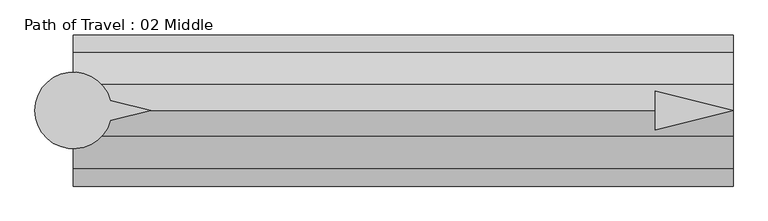
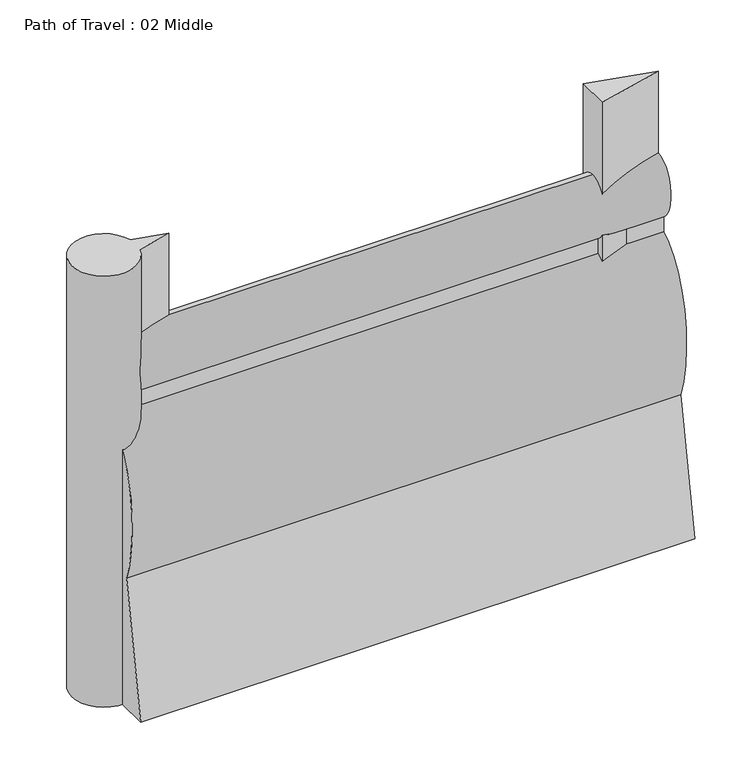
"""IFC4 building model written with IfcOpenShell, lengths in millimetres: proxy geometry, Path of Travel : 02 Middle."""

from ifc_helpers import new_model, si_unit, point, frame, frame_2d, origin, origin_with_axes, place, context, project, spatial, polyline, circle_curve, ellipse_curve, trimmed, segment, composite_curve, outline, extrude, source, transform, mapped, element, save
from ifc_brep_helpers import plane_surface, extruded_surface, advanced_brep


def path_of_travel_02_middle_c592e2b7(model_context):
    return source(origin(), model_context, "Body", "SolidModel", [
        advanced_brep(
        [(227.5554837, 0.0, 1727.2), (227.5554837, 42.9018657, 1436.6534209), (227.5554837, 42.9018657, 1363.4763406), (227.5554837, 184.1186263, 643.4144547), (227.5554837, 297.5699544, 0.0), (227.5554837, 145.6574193, 0.0), (227.5554837, 0.0, 584.2), (227.5554837, -145.6574193, 0.0), (227.5554837, -297.5699544, 0.0), (227.5554837, -184.1186263, 643.4144547), (227.5554837, -42.9018657, 1363.4763406), (227.5554837, -42.9018657, 1436.6534209), (2818.3554837, 0.0, 1727.2), (2818.3554837, -42.9018657, 1436.6534209), (2818.3554837, -42.9018657, 1363.4763406), (2818.3554837, -184.1186263, 643.4144547), (2818.3554837, -297.5699544, 0.0), (2818.3554837, -145.6574193, 0.0), (2818.3554837, 0.0, 584.2), (2818.3554837, 145.6574193, 0.0), (2818.3554837, 297.5699544, 0.0), (2818.3554837, 184.1186263, 643.4144547), (2818.3554837, 42.9018657, 1363.4763406), (2818.3554837, 42.9018657, 1436.6534209)],
        [
            (0, 1, ellipse_curve(frame((227.5554837, 0.0, 1574.8), z_axis=(-1.0, 0.0, 0.0), x_axis=(0.0, 0.0, 1.0)), 152.4, 101.6)),
            (1, 2),
            (2, 3, ellipse_curve(frame((227.5554837, 0.0, 914.4), z_axis=(-1.0, 0.0, 0.0), x_axis=(0.0, 0.0, -1.0)), 457.2, 228.6)),
            (3, 4),
            (4, 5),
            (5, 6),
            (6, 7),
            (7, 8),
            (8, 9),
            (9, 10, ellipse_curve(frame((227.5554837, 0.0, 914.4), z_axis=(-1.0, 0.0, 0.0), x_axis=(0.0, 0.0, -1.0)), 457.2, 228.6)),
            (10, 11),
            (11, 0, ellipse_curve(frame((227.5554837, 0.0, 1574.8), z_axis=(-1.0, 0.0, 0.0), x_axis=(0.0, 0.0, 1.0)), 152.4, 101.6)),
            (12, 13, ellipse_curve(frame((2818.3554837, 0.0, 1574.8), z_axis=(1.0, 0.0, 0.0), x_axis=(0.0, 0.0, 1.0)), 152.4, 101.6)),
            (13, 14),
            (14, 15, ellipse_curve(frame((2818.3554837, 0.0, 914.4), z_axis=(1.0, 0.0, 0.0), x_axis=(0.0, 0.0, -1.0)), 457.2, 228.6)),
            (15, 16),
            (16, 17),
            (17, 18),
            (18, 19),
            (19, 20),
            (20, 21),
            (21, 22, ellipse_curve(frame((2818.3554837, 0.0, 914.4), z_axis=(1.0, 0.0, 0.0), x_axis=(0.0, 0.0, -1.0)), 457.2, 228.6)),
            (22, 23),
            (23, 12, ellipse_curve(frame((2818.3554837, 0.0, 1574.8), z_axis=(1.0, 0.0, 0.0), x_axis=(0.0, 0.0, 1.0)), 152.4, 101.6)),
            (0, 12),
            (23, 1),
            (22, 2),
            (21, 3),
            (20, 4),
            (19, 5),
            (18, 6),
            (17, 7),
            (16, 8),
            (15, 9),
            (14, 10),
            (13, 11),
        ],
        [
            plane_surface(frame((227.5554837, 0.0, 0.0), z_axis=(-1.0, 0.0, 0.0), x_axis=(0.0, 0.0, 1.0))),
            plane_surface(frame((2818.3554837, 0.0, 0.0), z_axis=(1.0, 0.0, 0.0), x_axis=(0.0, 0.0, 1.0))),
            extruded_surface(trimmed(ellipse_curve(frame((2818.3554837, 0.0, 1574.8), z_axis=(-1.0, 0.0, 0.0), x_axis=(0.0, 0.0, 1.0)), 152.4, 101.6), [point((2818.3554837, 0.0, 1727.2))], [point((2818.3554837, 42.9018657, 1436.6534209))], True, "CARTESIAN"), (-2590.8, 0.0, 0.0), 2590.8),
            plane_surface(frame((227.5554837, 42.9018657, 1436.6534209), z_axis=(0.0, 1.0, 0.0), x_axis=(1.0, 0.0, 0.0))),
            extruded_surface(trimmed(ellipse_curve(frame((2818.3554837, 0.0, 914.4), z_axis=(-1.0, 0.0, 0.0), x_axis=(0.0, 0.0, -1.0)), 457.2, 228.6), [point((2818.3554837, 42.9018657, 1363.4763406))], [point((2818.3554837, 184.1186263, 643.4144547))], True, "CARTESIAN"), (-2590.8, 0.0, 0.0), 2590.8),
            plane_surface(frame((227.5554837, 184.1186263, 643.4144547), z_axis=(0.0, 0.9848077530122078, 0.1736481776669322), x_axis=(1.0, 0.0, 0.0))),
            plane_surface(frame((227.5554837, 297.5699544, 0.0), z_axis=(0.0, 0.0, -1.0), x_axis=(1.0, 0.0, 0.0))),
            plane_surface(frame((227.5554837, 145.6574193, 0.0), z_axis=(0.0, -0.9702957262760199, -0.2419218955995739), x_axis=(1.0, 0.0, 0.0))),
            plane_surface(frame((227.5554837, 0.0, 584.2), z_axis=(0.0, 0.9702957262759961, -0.24192189559966923), x_axis=(1.0, 0.0, 0.0))),
            plane_surface(frame((227.5554837, -145.6574193, 0.0), z_axis=(0.0, 0.0, -1.0), x_axis=(1.0, 0.0, 0.0))),
            plane_surface(frame((227.5554837, -297.5699544, 0.0), z_axis=(0.0, -0.984807753012208, 0.17364817766693066), x_axis=(1.0, 0.0, 0.0))),
            extruded_surface(trimmed(ellipse_curve(frame((2818.3554837, 0.0, 914.4), z_axis=(-1.0, 0.0, 0.0), x_axis=(0.0, 0.0, -1.0)), 457.2, 228.6), [point((2818.3554837, -184.1186263, 643.4144547))], [point((2818.3554837, -42.9018657, 1363.4763406))], True, "CARTESIAN"), (-2590.8, 0.0, 0.0), 2590.8),
            plane_surface(frame((227.5554837, -42.9018657, 1363.4763406), z_axis=(0.0, -1.0, 0.0), x_axis=(1.0, 0.0, 0.0))),
            extruded_surface(trimmed(ellipse_curve(frame((2818.3554837, 0.0, 1574.8), z_axis=(-1.0, 0.0, 0.0), x_axis=(0.0, 0.0, 1.0)), 152.4, 101.6), [point((2818.3554837, -42.9018657, 1436.6534209))], [point((2818.3554837, 0.0, 1727.2))], True, "CARTESIAN"), (-2590.8, 0.0, 0.0), 2590.8),
        ],
        [
            (0, [[1, 2, 3, 4, 5, 6, 7, 8, 9, 10, 11, 12]]),
            (1, [[13, 14, 15, 16, 17, 18, 19, 20, 21, 22, 23, 24]]),
            (2, [[-1, 25, -24, 26]]),
            (3, [[-2, -26, -23, 27]]),
            (4, [[-3, -27, -22, 28]]),
            (5, [[-4, -28, -21, 29]]),
            (6, [[-5, -29, -20, 30]]),
            (7, [[-6, -30, -19, 31]]),
            (8, [[-7, -31, -18, 32]]),
            (9, [[-8, -32, -17, 33]]),
            (10, [[-9, -33, -16, 34]]),
            (11, [[-10, -34, -15, 35]]),
            (12, [[-11, -35, -14, 36]]),
            (13, [[-12, -36, -13, -25]]),
        ],
    ),
        extrude(outline(polyline([(2512.3503371, 76.2006338), (2818.3554837, 0.0), (2512.3503371, -76.2006338), (2512.3503371, 76.2006338)])), origin_with_axes(), (0.0, 0.0, 1.0), 2129.5973753),
        extrude(outline(composite_curve([segment(polyline([(372.7837828, 39.4440225), (531.182385, 0.0), (372.7837828, -39.4440225)]), True, "CONTINUOUS"), segment(trimmed(circle_curve(frame_2d((227.2200886, 0.0)), 150.8131956), [point((372.7837828, -39.4440225))], [point((372.7837828, 39.4440225))], False, "CARTESIAN"), True, "CONTINUOUS")], self_intersect=False)), origin_with_axes(), (0.0, 0.0, 1.0), 2129.5973753),
    ])


if __name__ == "__main__":
    model = new_model("IFC4")
    model_context = context("Model", 3, world=origin())
    ifc_project = project(units=[si_unit("LENGTHUNIT", "METRE", prefix="MILLI")], contexts=[model_context])
    site = spatial("IfcSite", under=ifc_project)
    building = spatial("IfcBuilding", under=site)
    placement = place(None, origin())
    path_of_travel_02_middle_shape = path_of_travel_02_middle_c592e2b7(model_context)
    element("IfcBuildingElementProxy", 1, Name="Path of Travel : 02 Middle", ObjectType="Path of Travel : 02 Middle", at=placement, inside=building, context=model_context, shape_type="MappedRepresentation", body=[
        mapped(path_of_travel_02_middle_shape, transform((0.0, 0.0, 0.0), x_axis=(1.0, 0.0, 0.0), y_axis=(0.0, 1.0, 0.0), z_axis=(0.0, 0.0, 1.0))),
    ])
    save(model, "model.ifc")

# Revit data of these elements
# Type "Path of Travel : 02 Middle"
#   Path of Egress [instance default] = 4' - 0"
#   built-in parameter 1001306 [instance default] = 4 (stored number, unit not read)
#   Dot at Start = no
#   Arrow in Middle = yes
#   Arrow at End = no
#   Egress Path = none
# Element 1 (IfcBuildingElementProxy, "Path of Travel : 02 Middle")
#   Path of Egress = 8' - 6"
#   built-in parameter 1001306 = 8.5 (stored number, unit not read)
